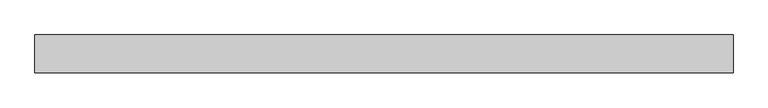
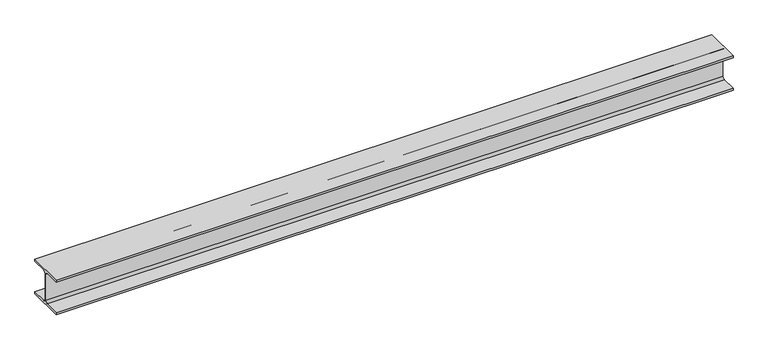
"""IFC4 building model written with IfcOpenShell, lengths in millimetres: beam geometry, 0912_Steel Framing_H-KSD3502 : H_SB_ASB_H-200x200x8x12."""

from ifc_helpers import new_model, si_unit, point, frame, frame_2d, origin, place, context, project, spatial, polyline, circle_curve, trimmed, segment, composite_curve, outline, extrude, source, transform, mapped, element, save


def beam_f311e2b4(model_context):
    return source(origin(), model_context, "Body", "SweptSolid", [
        extrude(outline(composite_curve([segment(polyline([(100.0, -88.0), (100.0, -100.0), (-100.0, -100.0), (-100.0, -88.0), (-17.0, -88.0)]), True, "CONTINUOUS"), segment(trimmed(circle_curve(frame_2d((-17.0, -75.0)), 13.0), [point((-17.0, -88.0))], [point((-4.0, -75.0))], True, "CARTESIAN"), True, "CONTINUOUS"), segment(polyline([(-4.0, -75.0), (-4.0, 75.0)]), True, "CONTINUOUS"), segment(trimmed(circle_curve(frame_2d((-17.0, 75.0)), 13.0), [point((-4.0, 75.0))], [point((-17.0, 88.0))], True, "CARTESIAN"), True, "CONTINUOUS"), segment(polyline([(-17.0, 88.0), (-100.0, 88.0), (-100.0, 100.0), (100.0, 100.0), (100.0, 88.0), (17.0, 88.0)]), True, "CONTINUOUS"), segment(trimmed(circle_curve(frame_2d((17.0, 75.0)), 13.0), [point((17.0, 88.0))], [point((4.0, 75.0))], True, "CARTESIAN"), True, "CONTINUOUS"), segment(polyline([(4.0, 75.0), (4.0, -75.0)]), True, "CONTINUOUS"), segment(trimmed(circle_curve(frame_2d((17.0, -75.0)), 13.0), [point((4.0, -75.0))], [point((17.0, -88.0))], True, "CARTESIAN"), True, "CONTINUOUS"), segment(polyline([(17.0, -88.0), (100.0, -88.0)]), True, "CONTINUOUS")], self_intersect=False)), frame((-1887.2000261, 0.0, 0.0), z_axis=(1.0, 0.0, 0.0), x_axis=(0.0, 1.0, 0.0)), (0.0, 0.0, 1.0), 3702.1907618),
    ])


if __name__ == "__main__":
    model = new_model("IFC4")
    model_context = context("Model", 3, world=origin())
    ifc_project = project(units=[si_unit("LENGTHUNIT", "METRE", prefix="MILLI")], contexts=[model_context])
    site = spatial("IfcSite", under=ifc_project)
    building = spatial("IfcBuilding", under=site)
    placement = place(None, origin())
    beam_shape = beam_f311e2b4(model_context)
    element("IfcBeam", 1, ObjectType="0912_Steel Framing_H-KSD3502 : H_SB_ASB_H-200x200x8x12", at=placement, inside=building, context=model_context, shape_type="MappedRepresentation", body=[
        mapped(beam_shape, transform((0.0, 0.0, 0.0), x_axis=(1.0, 0.0, 0.0), y_axis=(0.0, 1.0, 0.0), z_axis=(0.0, 0.0, 1.0))),
    ])
    save(model, "model.ifc")

# Revit data of these elements
# Type "0912_Steel Framing_H-KSD3502 : H_SB_ASB_H-200x200x8x12"
#   H_WM Code_1 = "S01AA002-00001 | Main Steel Structure Fabrication Work | Shelter/Building | Medium Steel - Standard (90KG/M>Weight≥30KG/M) | Material: (   )"
#   H_WM Code_2 = "S03AA028-00001 | Main Steel Structure Erection Work | Shelter/Building | Medium Steel (90KG/M>Weight≥30KG/M) | Material: (   )"
#   H_WM Code_3 = "S01AA010-00001 | Main Steel Structure Fabrication Work | Shelter/Building | Steel Painting/Coating | for Non-Fireproofed Steel Surface, Surface Preparation, Primer, Second & Final Coat | Material: (   )"
#   H_Q'ty Cal Type Tag = "SB-Q2"
#   Width = 20.0 cm
#   Web Thickness = 0.8 cm
#   Web Fillet = 1.3 cm
#   Warping Constant = 141000.0 cm⁶
#   W = 0
#   Torsional Moment of Inertia = 26.2485 cm⁴
#   Section Area = 63.53 cm²
#   Plastic Modulus weak axis = 244.0 cm³
#   Plastic Modulus strong axis = 525.0 cm³
#   Perimeter = 1.16 m²/m
#   Nominal Weight = 49.90 kgf/m
#   Moment of Inertia weak axis = 1600.00 cm⁴
#   Moment of Inertia strong axis = 4720.00 cm⁴
#   Height = 20.0 cm
#   Flange Thickness = 1.2 cm
#   Elastic Modulus weak axis = 160.0 cm³
#   Elastic Modulus strong axis = 472.0 cm³
#   Centroid Vertical = 10.0 cm
#   Centroid Horizontal = 10.0 cm
#   Ix = 47200000
#   Length [instance default] = 1.5240 m
#   Zx = 525000
#   b = 0.2000 m
#   h = 0.2000 m
#   r = 0.0130 m
#   s = 0.0080 m
#   t = 0.0120 m
#   A = 0.006353 m²
#   Structural Material [instance default] = Steel, 45-345
#   Assembly Code = ""
# Element 1 (IfcBeam, "0912_Steel Framing_H-KSD3502 : H_SB_ASB_H-200x200x8x12")
#   Structural Material = none
# Materials
#   "Steel, 45-345": class "Metal", colour RGB 189 187 185, transparency 0, Description = "Steel 345 MPa", Cost = 0
